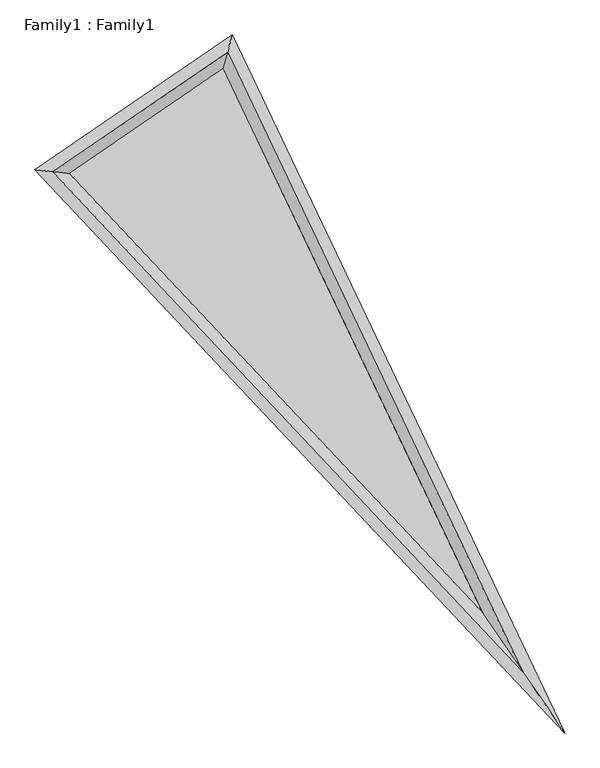
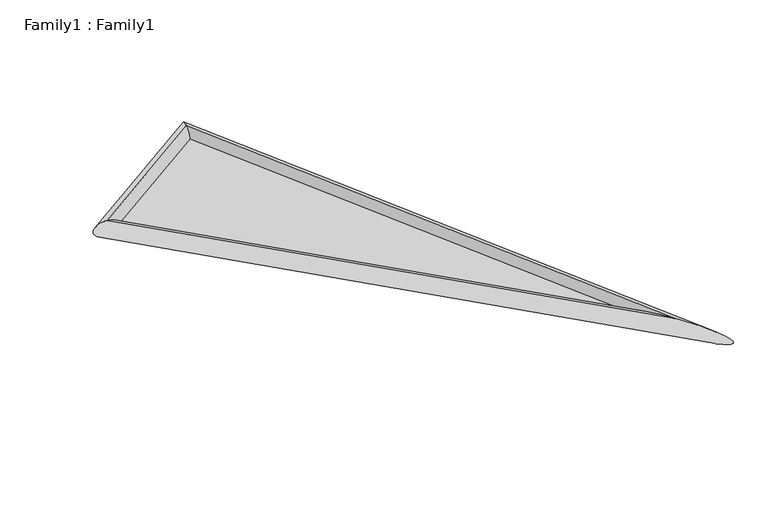
"""IFC4 building model written with IfcOpenShell, lengths in millimetres: proxy geometry, Family1 : Family1."""

from ifc_helpers import new_model, si_unit, frame, origin, origin_with_axes, place, context, project, spatial, polyline, ellipse_curve, outline, extrude, source, transform, mapped, element, save
from ifc_brep_helpers import cylinder_surface, advanced_brep


def family1_family1_9771ee4e(model_context):
    return source(origin(), model_context, "Body", "SolidModel", [
        extrude(outline(polyline([(3132.3574148, -2770.739152), (-940.8914968, 1558.9073162), (575.456533, 2595.7730408), (3132.3574148, -2770.739152)])), origin_with_axes(), (0.0, 0.0, 1.0), 34.1328789),
        advanced_brep(
        [(3132.3574148, -2770.739152, 100.0), (3132.3574148, -2770.739152, -100.0), (-940.8914968, 1558.9073162, -100.0), (-940.8914968, 1558.9073162, 100.0), (575.456533, 2595.7730408, -100.0), (575.456533, 2595.7730408, 100.0)],
        [
            (0, 1, ellipse_curve(frame((3132.3574148, -2770.739152, 0.0), z_axis=(-0.825468469717362, -0.56444823102077, 0.0), x_axis=(0.56444823102077, -0.825468469717362, 0.0)), 647.2135955, 100.0)),
            (1, 2),
            (2, 3, ellipse_curve(frame((-940.8914968, 1558.9073162, 0.0), z_axis=(-0.10785828638544533, -0.9941662788779326, 0.0), x_axis=(0.9941662788779326, -0.10785828638544526, 0.0)), 153.8014303, 100.0)),
            (3, 0),
            (1, 0, ellipse_curve(frame((3132.3574148, -2770.739152, 0.0), z_axis=(-0.825468469717362, -0.56444823102077, 0.0), x_axis=(0.56444823102077, -0.825468469717362, 0.0)), 647.2135955, 100.0)),
            (3, 2, ellipse_curve(frame((-940.8914968, 1558.9073162, 0.0), z_axis=(-0.10785828638544533, -0.9941662788779326, 0.0), x_axis=(0.9941662788779326, -0.10785828638544526, 0.0)), 153.8014303, 100.0)),
            (2, 4),
            (4, 5, ellipse_curve(frame((575.456533, 2595.7730408, 0.0), z_axis=(-0.9655627712424136, 0.26017020350276526, 0.0), x_axis=(-0.26017020350276526, -0.9655627712424136, 0.0)), 153.8014303, 100.0)),
            (5, 3),
            (5, 4, ellipse_curve(frame((575.456533, 2595.7730408, 0.0), z_axis=(-0.9655627712424136, 0.26017020350276526, 0.0), x_axis=(-0.26017020350276526, -0.9655627712424136, 0.0)), 153.8014303, 100.0)),
            (4, 1),
            (0, 5),
        ],
        [
            cylinder_surface(frame((3132.3574148, -2770.739152, 0.0), z_axis=(0.6852119243820388, -0.7283437503573866, 0.0), x_axis=(-0.7283437503573866, -0.6852119243820388, 0.0)), 100.0),
            cylinder_surface(frame((-940.8914968, 1558.9073162, 0.0), z_axis=(-0.8254684697173622, -0.5644482310207699, 0.0), x_axis=(-0.5644482310207699, 0.8254684697173622, 0.0)), 100.0),
            cylinder_surface(frame((575.456533, 2595.7730408, 0.0), z_axis=(-0.43012813891869806, 0.902767846187677, 0.0), x_axis=(0.902767846187677, 0.43012813891869806, 0.0)), 100.0),
        ],
        [
            (0, [[1, 2, 3, 4]]),
            (0, [[5, -4, 6, -2]]),
            (1, [[-3, 7, 8, 9]]),
            (1, [[-6, -9, 10, -7]]),
            (2, [[-8, 11, -1, 12]]),
            (2, [[-10, -12, -5, -11]]),
        ],
    ),
    ])


if __name__ == "__main__":
    model = new_model("IFC4")
    model_context = context("Model", 3, world=origin())
    ifc_project = project(units=[si_unit("LENGTHUNIT", "METRE", prefix="MILLI")], contexts=[model_context])
    site = spatial("IfcSite", under=ifc_project)
    building = spatial("IfcBuilding", under=site)
    placement = place(None, origin())
    family1_family1_shape = family1_family1_9771ee4e(model_context)
    element("IfcBuildingElementProxy", 1, Name="Family1 : Family1", ObjectType="Family1 : Family1", at=placement, inside=building, context=model_context, shape_type="MappedRepresentation", body=[
        mapped(family1_family1_shape, transform((0.0, 0.0, 0.0), x_axis=(1.0, 0.0, 0.0), y_axis=(0.0, 1.0, 0.0), z_axis=(0.0, 0.0, 1.0))),
    ])
    save(model, "model.ifc")

# Revit data of these elements
# Type "Family1 : Family1"
#   Default Elevation = 0
# Element 1 (IfcBuildingElementProxy, "Family1 : Family1")
#   Materials on its faces: "Glass"
# Materials
#   "Glass": class "Glass", colour RGB 0 128 192, transparency 0.9, Description = "Soda Lime Glass", Cost = 0
